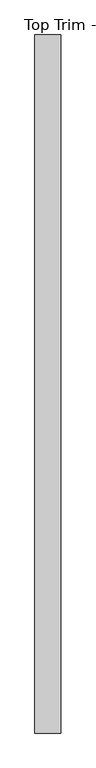
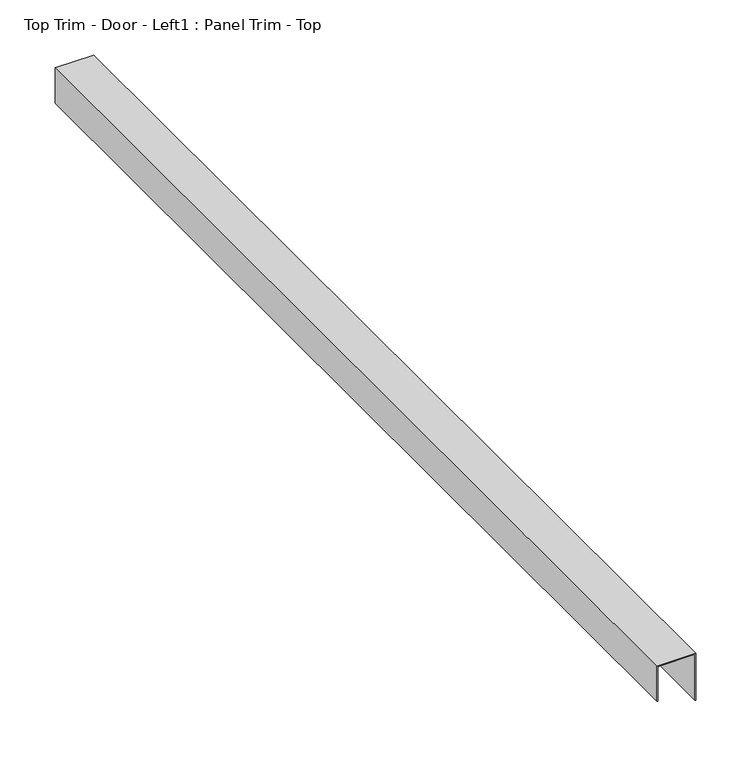
"""IFC4 building model written with IfcOpenShell, lengths in millimetres: proxy geometry, Top Trim - Door - Left1 : Panel Trim - Top."""

from ifc_helpers import new_model, si_unit, frame, origin, place, context, project, spatial, polyline, outline, extrude, source, transform, mapped, element, save


def top_trim_door_left1_panel_trim_top_50f9c082(model_context):
    return source(origin(), model_context, "Body", "SweptSolid", [
        extrude(outline(polyline([(2438.4, 587327.0060739), (2438.4, 587365.8934739), (2387.6, 587365.8934739), (2387.6, 587366.6808739), (2439.19375, 587366.6808739), (2439.19375, 587326.2186739), (2400.3, 587326.2186739), (2400.3, 587327.0060739), (2438.4, 587327.0060739)])), frame((0.0, -535201.5663841, 0.0), z_axis=(0.0, 1.0, 0.0), x_axis=(0.0, 0.0, 1.0)), (0.0, 0.0, 1.0), 1092.2),
    ])


if __name__ == "__main__":
    model = new_model("IFC4")
    model_context = context("Model", 3, world=origin())
    ifc_project = project(units=[si_unit("LENGTHUNIT", "METRE", prefix="MILLI")], contexts=[model_context])
    site = spatial("IfcSite", under=ifc_project)
    building = spatial("IfcBuilding", under=site)
    placement = place(None, origin())
    top_trim_door_left1_panel_trim_top_shape = top_trim_door_left1_panel_trim_top_50f9c082(model_context)
    element("IfcBuildingElementProxy", 1, Name="Top Trim - Door - Left1 : Panel Trim - Top", ObjectType="Top Trim - Door - Left1 : Panel Trim - Top", at=placement, inside=building, context=model_context, shape_type="MappedRepresentation", body=[
        mapped(top_trim_door_left1_panel_trim_top_shape, transform((0.0, 0.0, 0.0), x_axis=(1.0, 0.0, 0.0), y_axis=(0.0, 1.0, 0.0), z_axis=(0.0, 0.0, 1.0))),
    ])
    save(model, "model.ifc")

# Revit data of these elements
# Element 1 (IfcBuildingElementProxy, "Top Trim - Door - Left1 : Panel Trim - Top")
#   Materials on its faces: "EDGE TRIM BY MTL PANEL MFR."
# Materials
#   "EDGE TRIM BY MTL PANEL MFR.": class "Generic", colour RGB 239 242 240, transparency 0, Cost = 0
